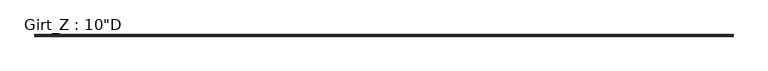
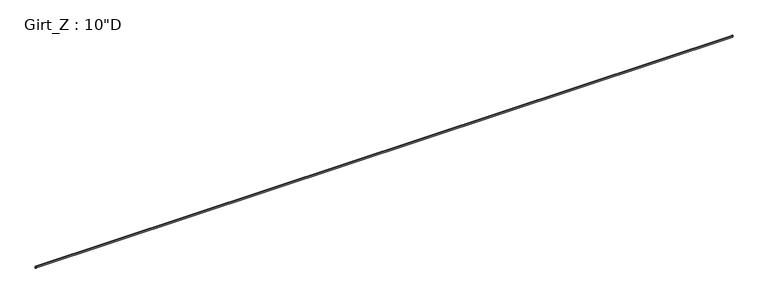
"""IFC4 building model written with IfcOpenShell, lengths in millimetres: beam geometry."""

from ifc_helpers import new_model, si_unit, point, frame, frame_2d, origin, place, context, project, spatial, polyline, circle_curve, trimmed, segment, composite_curve, outline, extrude, source, transform, mapped, element, save


def beam_b320f09e(model_context):
    return source(origin(), model_context, "Body", "SweptSolid", [
        extrude(outline(composite_curve([segment(polyline([(-77.9859375, 127.0), (-3.3734375, 127.0)]), True, "CONTINUOUS"), segment(trimmed(circle_curve(frame_2d((-3.3734375, 122.2375)), 4.7625), [point((-3.3734375, 127.0))], [point((1.3890625, 122.2375))], False, "CARTESIAN"), True, "CONTINUOUS"), segment(polyline([(1.3890625, 122.2375), (1.3890625, -122.2389339)]), True, "CONTINUOUS"), segment(trimmed(circle_curve(frame_2d((3.3748024, -122.2389339)), 1.9857399), [point((1.3890625, -122.2389339))], [point((3.2694106, -124.221875))], True, "CARTESIAN"), True, "CONTINUOUS"), segment(polyline([(3.2694106, -124.221875), (83.0404765, -124.221875), (94.4528742, -110.621109), (96.5810415, -112.4068534), (84.3359375, -127.0), (-1.3890625, -127.0), (-1.3890625, 122.2381931)]), True, "CONTINUOUS"), segment(trimmed(circle_curve(frame_2d((-3.3741066, 122.2381931)), 1.9850441), [point((-1.3890625, 122.2381931))], [point((-3.3005807, 124.221875))], True, "CARTESIAN"), True, "CONTINUOUS"), segment(polyline([(-3.3005807, 124.221875), (-76.6904765, 124.221875), (-88.1028742, 110.621109), (-90.2310415, 112.4068534), (-77.9859375, 127.0)]), True, "CONTINUOUS")], self_intersect=False)), frame((-40544.2674, 0.0, 0.0), z_axis=(1.0, 0.0, 0.0), x_axis=(0.0, 1.0, 0.0)), (0.0, 0.0, 1.0), 81158.969),
    ])


if __name__ == "__main__":
    model = new_model("IFC4")
    model_context = context("Model", 3, world=origin())
    ifc_project = project(units=[si_unit("LENGTHUNIT", "METRE", prefix="MILLI")], contexts=[model_context])
    site = spatial("IfcSite", under=ifc_project)
    building = spatial("IfcBuilding", under=site)
    placement = place(None, origin())
    beam_shape = beam_b320f09e(model_context)
    element("IfcBeam", 1, ObjectType="Girt_Z : 10\"D", at=placement, inside=building, context=model_context, shape_type="MappedRepresentation", body=[
        mapped(beam_shape, transform((0.0, 0.0, 0.0), x_axis=(1.0, 0.0, 0.0), y_axis=(0.0, 1.0, 0.0), z_axis=(0.0, 0.0, 1.0))),
    ])
    save(model, "model.ifc")

# Revit data of these elements
# Type "Girt_Z : 10\"D"
#   half leg = 0' - 1 11/16"
#   Web_Thickness = 0' - 0 7/64"
#   Length [instance default] = 10' - 0"
#   Leg_2 = 0' - 3 3/8"
#   Leg_1 = 0' - 3 1/8"
#   Height = 0' - 10"
#   Structural Material [instance default] = none
